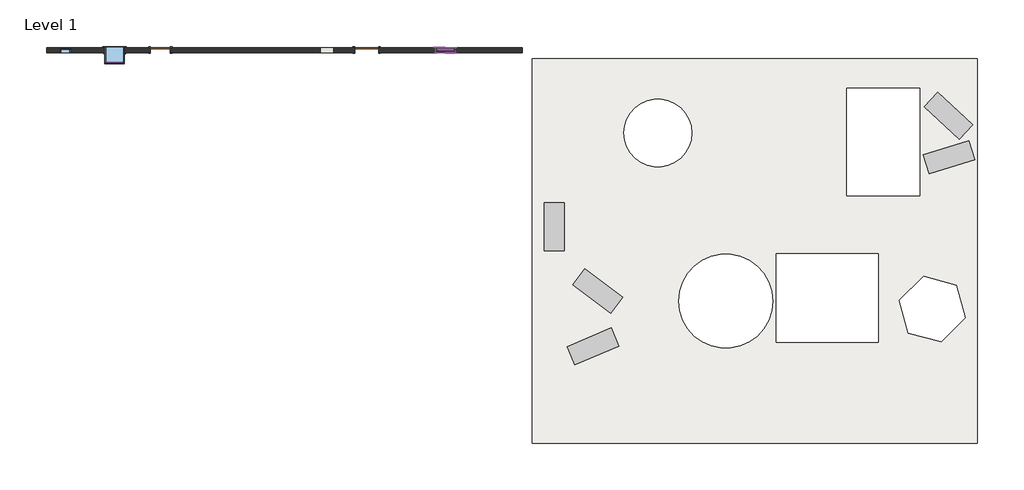
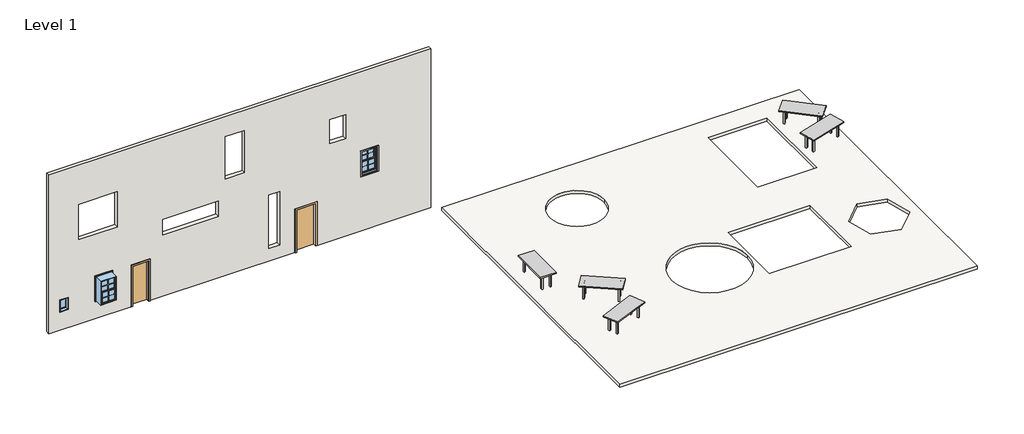
# One storey: 8 furniture elements, 8 proxies, 3 windows, 2 doors, 2 slabs, 1 wall.
"""IFC4 building model written with IfcOpenShell, lengths in millimetres."""

import ifcopenshell
import ifcopenshell.guid

model = None  # the IFC model being written
_history = None  # IfcOwnerHistory: only IFC2X3 demands one
_inside = {}  # id of a spatial element -> (the spatial element, [elements in it])
_under = {}  # id of a project, library or spatial element -> (it, [spatial elements below it])
_declared = {}  # id of a project -> (the project, [libraries it declares])
_typed = {}  # id of a type object -> (the type object, [elements of that type])
_made_of = {}  # id of a material, layer set ... -> (it, [elements and type objects made of it])


def new_model(schema):
    """Start an empty IFC model of exactly this schema.

    Asked for "IFC4X3", IfcOpenShell would pick the latest addendum, in which some entities
    have other attributes; the version numbers below select the first issue.
    IFC2X3 requires an IfcOwnerHistory on every rooted entity: one is made here for all.
    """
    global model, _history
    if schema == "IFC4X3":
        model = ifcopenshell.file(schema_version=(4, 3, 0, 0))
    else:
        model = ifcopenshell.file(schema=schema)
    _inside.clear()
    _under.clear()
    _declared.clear()
    _typed.clear()
    _made_of.clear()
    _history = None
    if model.schema == "IFC2X3":
        org = make("IfcOrganization", Name="unknown")
        user = make(
            "IfcPersonAndOrganization",
            ThePerson=make("IfcPerson", FamilyName="unknown"),
            TheOrganization=org,
        )
        app = make(
            "IfcApplication",
            ApplicationDeveloper=org,
            Version="unknown",
            ApplicationFullName="unknown",
            ApplicationIdentifier="unknown",
        )
        _history = make(
            "IfcOwnerHistory",
            OwningUser=user,
            OwningApplication=app,
            ChangeAction="ADDED",
            CreationDate=0,
        )
    return model


def make(cls, **values):
    """One entity of the class cls with the attributes given. An attribute that is None is left unset."""
    return model.create_entity(
        cls, **{name: value for name, value in values.items() if value is not None}
    )


def rooted(cls, **values):
    """An entity with a GlobalId (a new one), such as an element, a storey or a relation."""
    return make(cls, GlobalId=ifcopenshell.guid.new(), OwnerHistory=_history, **values)


def si_unit(unit_type, name, prefix=None):
    """IfcSIUnit, for example si_unit("LENGTHUNIT", "METRE", prefix="MILLI")."""
    return make("IfcSIUnit", UnitType=unit_type, Prefix=prefix, Name=name)


def assignment(units):
    """IfcUnitAssignment: the units of a project."""
    return None if units is None else make("IfcUnitAssignment", Units=units)


def point(xyz):
    """IfcCartesianPoint."""
    return None if xyz is None else make("IfcCartesianPoint", Coordinates=xyz)


def direction(xyz):
    """IfcDirection."""
    return None if xyz is None else make("IfcDirection", DirectionRatios=xyz)


def frame(location, z_axis=None, x_axis=None):
    """IfcAxis2Placement3D, a coordinate frame: its origin and axes. An axis left out is left unset."""
    return make(
        "IfcAxis2Placement3D",
        Location=point(location),
        Axis=direction(z_axis),
        RefDirection=direction(x_axis),
    )


def frame_2d(location, x_axis=None):
    """IfcAxis2Placement2D, a coordinate frame in the plane: its origin and x axis."""
    return make(
        "IfcAxis2Placement2D", Location=point(location), RefDirection=direction(x_axis)
    )


def origin():
    """The frame at (0, 0, 0) with its axes left unset."""
    return frame((0.0, 0.0, 0.0))


def origin_with_axes():
    """The frame at (0, 0, 0) with the z axis (0, 0, 1) and the x axis (1, 0, 0) written out."""
    return frame((0.0, 0.0, 0.0), z_axis=(0.0, 0.0, 1.0), x_axis=(1.0, 0.0, 0.0))


def place(relative_to, where):
    """IfcLocalPlacement: puts the frame where relative to a parent placement (None: the world)."""
    return make(
        "IfcLocalPlacement", PlacementRelTo=relative_to, RelativePlacement=where
    )


def context(
    kind, dimensions, precision=None, world=None, true_north=None, identifier=None
):
    """IfcGeometricRepresentationContext, for example the 3D "Model" context."""
    return make(
        "IfcGeometricRepresentationContext",
        ContextIdentifier=identifier,
        ContextType=kind,
        CoordinateSpaceDimension=dimensions,
        Precision=precision,
        WorldCoordinateSystem=world,
        TrueNorth=true_north,
    )


def project(units=None, contexts=None):
    """IfcProject with its units and contexts."""
    return rooted(
        "IfcProject",
        Name="project",
        RepresentationContexts=contexts,
        UnitsInContext=assignment(units),
    )


def spatial(cls, under=None, at=None, **own):
    """A site, building, storey or space (cls), placed at a placement, below another one or the project."""
    s = rooted(cls, ObjectPlacement=at, **own)
    if under is not None:
        _under.setdefault(under.id(), (under, []))[1].append(s)
    return s


def polyline(points):
    """IfcPolyline through the points."""
    return make("IfcPolyline", Points=[point(p) for p in points])


def circle_curve(where, radius):
    """IfcCircle in the frame where."""
    return make("IfcCircle", Position=where, Radius=radius)


def trimmed(basis, trim1, trim2, sense, master):
    """IfcTrimmedCurve: the piece of a basis curve between two trims."""
    return make(
        "IfcTrimmedCurve",
        BasisCurve=basis,
        Trim1=trim1,
        Trim2=trim2,
        SenseAgreement=sense,
        MasterRepresentation=master,
    )


def segment(curve, same_sense, transition):
    """IfcCompositeCurveSegment."""
    return make(
        "IfcCompositeCurveSegment",
        Transition=transition,
        SameSense=same_sense,
        ParentCurve=curve,
    )


def composite_curve(segments, self_intersect=None):
    """IfcCompositeCurve: segments joined end to end."""
    return make("IfcCompositeCurve", Segments=segments, SelfIntersect=self_intersect)


def outline(outer, holes=None, kind="AREA"):
    """IfcArbitraryClosedProfileDef: a profile drawn as a closed curve; with holes, ...WithVoids."""
    if holes is None:
        return make("IfcArbitraryClosedProfileDef", ProfileType=kind, OuterCurve=outer)
    return make(
        "IfcArbitraryProfileDefWithVoids",
        ProfileType=kind,
        OuterCurve=outer,
        InnerCurves=holes,
    )


def extrude(swept, where, along, depth):
    """IfcExtrudedAreaSolid: the profile swept, set in the frame where, extruded along a direction by depth."""
    return make(
        "IfcExtrudedAreaSolid",
        SweptArea=swept,
        Position=where,
        ExtrudedDirection=direction(along),
        Depth=depth,
    )


def shape(context_of_items, identifier, shape_type, items):
    """IfcShapeRepresentation: the items that make up one representation, for example the "Body"."""
    return make(
        "IfcShapeRepresentation",
        ContextOfItems=context_of_items,
        RepresentationIdentifier=identifier,
        RepresentationType=shape_type,
        Items=items,
    )


def source(mapping_origin, context_of_items, identifier, shape_type, items):
    """IfcRepresentationMap: a shape defined once, which mapped items show again and again."""
    return make(
        "IfcRepresentationMap",
        MappingOrigin=mapping_origin,
        MappedRepresentation=shape(context_of_items, identifier, shape_type, items),
    )


def transform(
    local_origin,
    x_axis=None,
    y_axis=None,
    z_axis=None,
    scale=None,
    scale2=None,
    scale3=None,
    uniform=True,
):
    """IfcCartesianTransformationOperator3D, or its non-uniform kind. x_axis, y_axis, z_axis: its Axis1, 2, 3."""
    if uniform:
        return make(
            "IfcCartesianTransformationOperator3D",
            Axis1=direction(x_axis),
            Axis2=direction(y_axis),
            LocalOrigin=point(local_origin),
            Scale=scale,
            Axis3=direction(z_axis),
        )
    return make(
        "IfcCartesianTransformationOperator3DnonUniform",
        Axis1=direction(x_axis),
        Axis2=direction(y_axis),
        LocalOrigin=point(local_origin),
        Scale=scale,
        Axis3=direction(z_axis),
        Scale2=scale2,
        Scale3=scale3,
    )


def mapped(mapping_source, mapping_target):
    """IfcMappedItem: shows the shape of a source again, moved by a transform."""
    return make(
        "IfcMappedItem", MappingSource=mapping_source, MappingTarget=mapping_target
    )


def made_of(thing, what):
    """Note that an element or type object is made of a material, layer set ...; save() writes the relation."""
    if what is not None:
        _made_of.setdefault(what.id(), (what, []))[1].append(thing)
    return thing


def element(
    cls,
    number,
    at=None,
    inside=None,
    cuts=None,
    type_object=None,
    material=None,
    context=None,
    identifier="Body",
    shape_type=None,
    held_by="IfcProductDefinitionShape",
    body=None,
    shapes=None,
    **own,
):
    """One element of the class cls, such as IfcWall. Its Tag is "e" and its number.

    at: its placement. inside: the storey or other place that contains it. cuts: it is an
    opening in that element (IfcRelVoidsElement). A single representation is given by context,
    identifier, shape_type and body (its items); several are given by shapes. held_by: the class
    of the entity that holds the representations. save() writes the other relations.
    """
    e = rooted(cls, Tag="e%d" % number, ObjectPlacement=at, **own)
    if body is not None:
        shapes = [shape(context, identifier, shape_type, body)]
    if shapes is not None:
        e.Representation = make(held_by, Representations=shapes)
    if inside is not None:
        _inside.setdefault(inside.id(), (inside, []))[1].append(e)
    if cuts is not None:
        rooted(
            "IfcRelVoidsElement", RelatingBuildingElement=cuts, RelatedOpeningElement=e
        )
    if type_object is not None:
        _typed.setdefault(type_object.id(), (type_object, []))[1].append(e)
    return made_of(e, material)


def aggregate(whole, parts):
    """IfcRelAggregates: a whole, such as a stair, and the parts it consists of."""
    return rooted("IfcRelAggregates", RelatingObject=whole, RelatedObjects=parts)


def save(model, path):
    """Write the relations noted so far, then the file.

    IfcRelAggregates (storeys below a building ...), IfcRelContainedInSpatialStructure (elements
    in a storey), IfcRelDefinesByType, IfcRelAssociatesMaterial and IfcRelDeclares: one each for
    every whole, place, type object, material and project.
    """
    for whole, parts in _under.values():
        aggregate(whole, parts)
    for where, things in _inside.values():
        rooted(
            "IfcRelContainedInSpatialStructure",
            RelatedElements=things,
            RelatingStructure=where,
        )
    for kind, things in _typed.values():
        rooted("IfcRelDefinesByType", RelatedObjects=things, RelatingType=kind)
    for what, things in _made_of.values():
        rooted("IfcRelAssociatesMaterial", RelatedObjects=things, RelatingMaterial=what)
    for by, libraries in _declared.values():
        rooted("IfcRelDeclares", RelatingContext=by, RelatedDefinitions=libraries)
    model.write(path)


def m_muntin_pattern_2x2_m_muntin_pattern_2x2_aaec3afb(model_context):
    return source(origin(), model_context, "Body", "SweptSolid", [
        extrude(outline(polyline([(257.1375, -6.35), (257.1375, -298.8), (244.4375, -298.8), (244.4375, -6.35), (0.0, -6.35), (0.0, 6.35), (244.4375, 6.35), (244.4375, 298.8), (257.1375, 298.8), (257.1375, 6.35), (501.575, 6.35), (501.575, -6.35), (257.1375, -6.35)])), frame((0.0, 9.525, 0.0), z_axis=(0.0, 1.0, 0.0), x_axis=(0.0, 0.0, 1.0)), (0.0, 0.0, 1.0), 12.7),
        extrude(outline(polyline([(257.1375, -6.35), (257.1375, -298.8), (244.4375, -298.8), (244.4375, -6.35), (0.0, -6.35), (0.0, 6.35), (244.4375, 6.35), (244.4375, 298.8), (257.1375, 298.8), (257.1375, 6.35), (501.575, 6.35), (501.575, -6.35), (257.1375, -6.35)])), frame((0.0, -22.225, 0.0), z_axis=(0.0, 1.0, 0.0), x_axis=(0.0, 0.0, 1.0)), (0.0, 0.0, 1.0), 12.7),
    ])


def m_trim_window_exterior_flat_with_sill_e7ff6350(model_context):
    return source(origin(), model_context, "Body", "SweptSolid", [
        extrude(outline(polyline([(435.0, -1220.4323709), (435.0, -1280.4323709), (-435.0, -1280.4323709), (-435.0, -1220.4323709), (435.0, -1220.4323709)])), origin_with_axes(), (0.0, 0.0, 1.0), 19.05),
        extrude(outline(polyline([(-1230.0, 38.1), (-1202.4580645, 38.1), (-1200.0, 19.05), (-1200.0, 0.0), (-1220.4323709, 0.0), (-1220.4323709, 19.05), (-1230.0, 19.05), (-1230.0, 38.1)])), frame((-447.7, 0.0, 0.0), z_axis=(1.0, 0.0, 0.0), x_axis=(0.0, 1.0, 0.0)), (0.0, 0.0, 1.0), 895.4),
        extrude(outline(polyline([(-435.0, 60.0), (435.0, 60.0), (435.0, -1200.0), (375.0, -1200.0), (375.0, 0.0), (-375.0, 0.0), (-375.0, -1200.0), (-435.0, -1200.0), (-435.0, 60.0)])), origin_with_axes(), (0.0, 0.0, 1.0), 19.05),
    ])


def m_trim_window_interior_flat_picture_frame_31bd2320(model_context):
    return source(origin(), model_context, "Body", "SweptSolid", [
        extrude(outline(polyline([(422.3, 47.3), (422.3, -1247.3), (-422.3, -1247.3), (-422.3, 47.3), (422.3, 47.3)]), holes=[polyline([(362.3, -12.7), (-362.3, -12.7), (-362.3, -1187.3), (362.3, -1187.3), (362.3, -12.7)])]), origin_with_axes(), (0.0, 0.0, 1.0), 30.0),
    ])


def m_single_flush_0762_x_2032mm_0c256fab(model_context):
    return source(origin(), model_context, "Body", "SweptSolid", [
        extrude(outline(polyline([(2108.0, -457.0), (0.0, -457.0), (0.0, -381.0), (2032.0, -381.0), (2032.0, 381.0), (0.0, 381.0), (0.0, 457.0), (2108.0, 457.0), (2108.0, -457.0)])), frame((0.0, 100.0, 0.0), z_axis=(0.0, 1.0, 0.0), x_axis=(0.0, 0.0, 1.0)), (0.0, 0.0, 1.0), 25.0),
        extrude(outline(polyline([(2108.0, 457.0), (2108.0, -457.0), (0.0, -457.0), (0.0, -381.0), (2032.0, -381.0), (2032.0, 381.0), (0.0, 381.0), (0.0, 457.0), (2108.0, 457.0)])), frame((0.0, -125.0, 0.0), z_axis=(0.0, 1.0, 0.0), x_axis=(0.0, 0.0, 1.0)), (0.0, 0.0, 1.0), 25.0),
        extrude(outline(polyline([(381.0, 49.0), (-381.0, 49.0), (-381.0, 100.0), (381.0, 100.0), (381.0, 49.0)])), origin_with_axes(), (0.0, 0.0, 1.0), 2032.0),
    ])


def m_single_flush_0915_x_2134mm_727434cd(model_context):
    return source(origin(), model_context, "Body", "SweptSolid", [
        extrude(outline(polyline([(2210.0, -533.5), (0.0, -533.5), (0.0, -457.5), (2134.0, -457.5), (2134.0, 457.5), (0.0, 457.5), (0.0, 533.5), (2210.0, 533.5), (2210.0, -533.5)])), frame((0.0, -125.0, 0.0), z_axis=(0.0, 1.0, 0.0), x_axis=(0.0, 0.0, 1.0)), (0.0, 0.0, 1.0), 25.0),
        extrude(outline(polyline([(2210.0, 533.5), (2210.0, -533.5), (0.0, -533.5), (0.0, -457.5), (2134.0, -457.5), (2134.0, 457.5), (0.0, 457.5), (0.0, 533.5), (2210.0, 533.5)])), frame((0.0, 100.0, 0.0), z_axis=(0.0, 1.0, 0.0), x_axis=(0.0, 0.0, 1.0)), (0.0, 0.0, 1.0), 25.0),
        extrude(outline(polyline([(457.5, -49.0), (457.5, -100.0), (-457.5, -100.0), (-457.5, -49.0), (457.5, -49.0)])), origin_with_axes(), (0.0, 0.0, 1.0), 2134.0),
    ])


def m_table_rectangular_1830_x_0762mm_a0b3b7a0(model_context):
    return source(origin(), model_context, "Body", "SweptSolid", [
        extrude(outline(polyline([(699.1, 190.5), (699.1, 165.1), (-699.1, 165.1), (-699.1, 190.5), (699.1, 190.5)])), frame((0.0, 0.0, 609.6), z_axis=(0.0, 0.0, 1.0), x_axis=(1.0, 0.0, 0.0)), (0.0, 0.0, 1.0), 101.6),
        extrude(outline(polyline([(699.1, -190.5), (-699.1, -190.5), (-699.1, -165.1), (699.1, -165.1), (699.1, -190.5)])), frame((0.0, 0.0, 609.6), z_axis=(0.0, 0.0, 1.0), x_axis=(1.0, 0.0, 0.0)), (0.0, 0.0, 1.0), 101.6),
        extrude(outline(polyline([(-711.8, -165.1), (-737.2, -165.1), (-737.2, 165.1), (-711.8, 165.1), (-711.8, -165.1)])), frame((0.0, 0.0, 609.6), z_axis=(0.0, 0.0, 1.0), x_axis=(1.0, 0.0, 0.0)), (0.0, 0.0, 1.0), 101.6),
        extrude(outline(polyline([(711.8, -165.1), (711.8, 165.1), (737.2, 165.1), (737.2, -165.1), (711.8, -165.1)])), frame((0.0, 0.0, 609.6), z_axis=(0.0, 0.0, 1.0), x_axis=(1.0, 0.0, 0.0)), (0.0, 0.0, 1.0), 101.6),
        extrude(outline(polyline([(915.0, 381.0), (915.0, -381.0), (-915.0, -381.0), (-915.0, 381.0), (915.0, 381.0)])), frame((0.0, 0.0, 711.2), z_axis=(0.0, 0.0, 1.0), x_axis=(1.0, 0.0, 0.0)), (0.0, 0.0, 1.0), 50.8),
        extrude(outline(polyline([(-699.1, 228.6), (-699.1, 165.1), (-762.6, 165.1), (-762.6, 228.6), (-699.1, 228.6)])), origin_with_axes(), (0.0, 0.0, 1.0), 711.2),
        extrude(outline(polyline([(699.1, 228.6), (762.6, 228.6), (762.6, 165.1), (699.1, 165.1), (699.1, 228.6)])), origin_with_axes(), (0.0, 0.0, 1.0), 711.2),
        extrude(outline(polyline([(-699.1, -228.6), (-762.6, -228.6), (-762.6, -165.1), (-699.1, -165.1), (-699.1, -228.6)])), origin_with_axes(), (0.0, 0.0, 1.0), 711.2),
        extrude(outline(polyline([(699.1, -228.6), (699.1, -165.1), (762.6, -165.1), (762.6, -228.6), (699.1, -228.6)])), origin_with_axes(), (0.0, 0.0, 1.0), 711.2),
    ])


def m_table_rectangular_1830_x_0762mm_ec068ed4(model_context):
    return source(origin(), model_context, "Body", "SweptSolid", [
        extrude(outline(polyline([(699.1, -190.5), (-699.1, -190.5), (-699.1, -165.1), (699.1, -165.1), (699.1, -190.5)])), frame((0.0, 0.0, 609.6), z_axis=(0.0, 0.0, 1.0), x_axis=(1.0, 0.0, 0.0)), (0.0, 0.0, 1.0), 101.6),
        extrude(outline(polyline([(699.1, 190.5), (699.1, 165.1), (-699.1, 165.1), (-699.1, 190.5), (699.1, 190.5)])), frame((0.0, 0.0, 609.6), z_axis=(0.0, 0.0, 1.0), x_axis=(1.0, 0.0, 0.0)), (0.0, 0.0, 1.0), 101.6),
        extrude(outline(polyline([(-711.8, 165.1), (-711.8, -165.1), (-737.2, -165.1), (-737.2, 165.1), (-711.8, 165.1)])), frame((0.0, 0.0, 609.6), z_axis=(0.0, 0.0, 1.0), x_axis=(1.0, 0.0, 0.0)), (0.0, 0.0, 1.0), 101.6),
        extrude(outline(polyline([(711.8, 165.1), (737.2, 165.1), (737.2, -165.1), (711.8, -165.1), (711.8, 165.1)])), frame((0.0, 0.0, 609.6), z_axis=(0.0, 0.0, 1.0), x_axis=(1.0, 0.0, 0.0)), (0.0, 0.0, 1.0), 101.6),
        extrude(outline(polyline([(915.0, -381.0), (-915.0, -381.0), (-915.0, 381.0), (915.0, 381.0), (915.0, -381.0)])), frame((0.0, 0.0, 711.2), z_axis=(0.0, 0.0, 1.0), x_axis=(1.0, 0.0, 0.0)), (0.0, 0.0, 1.0), 50.8),
        extrude(outline(polyline([(-699.1, -228.6), (-762.6, -228.6), (-762.6, -165.1), (-699.1, -165.1), (-699.1, -228.6)])), origin_with_axes(), (0.0, 0.0, 1.0), 711.2),
        extrude(outline(polyline([(699.1, -228.6), (699.1, -165.1), (762.6, -165.1), (762.6, -228.6), (699.1, -228.6)])), origin_with_axes(), (0.0, 0.0, 1.0), 711.2),
        extrude(outline(polyline([(-699.1, 228.6), (-699.1, 165.1), (-762.6, 165.1), (-762.6, 228.6), (-699.1, 228.6)])), origin_with_axes(), (0.0, 0.0, 1.0), 711.2),
        extrude(outline(polyline([(699.1, 228.6), (762.6, 228.6), (762.6, 165.1), (699.1, 165.1), (699.1, 228.6)])), origin_with_axes(), (0.0, 0.0, 1.0), 711.2),
    ])


def m_fixed_0406_x_0610mm_8205b201(model_context):
    return source(origin(), model_context, "Body", "SweptSolid", [
        extrude(outline(polyline([(-140.0, 78.0), (140.0, 78.0), (140.0, 66.0), (-140.0, 66.0), (-140.0, 78.0)])), frame((0.0, 0.0, 978.0), z_axis=(0.0, 0.0, 1.0), x_axis=(1.0, 0.0, 0.0)), (0.0, 0.0, 1.0), 484.0),
        extrude(outline(polyline([(1506.0, -184.0), (934.0, -184.0), (934.0, 184.0), (1506.0, 184.0), (1506.0, -184.0)]), holes=[polyline([(1462.0, -140.0), (1462.0, 140.0), (978.0, 140.0), (978.0, -140.0), (1462.0, -140.0)])]), frame((0.0, 50.0, 0.0), z_axis=(0.0, 1.0, 0.0), x_axis=(0.0, 0.0, 1.0)), (0.0, 0.0, 1.0), 44.0),
        extrude(outline(polyline([(1525.0, -203.0), (915.0, -203.0), (915.0, 203.0), (1525.0, 203.0), (1525.0, -203.0)]), holes=[polyline([(1506.0, -184.0), (1506.0, 184.0), (934.0, 184.0), (934.0, -184.0), (1506.0, -184.0)])]), frame((0.0, 50.0, 0.0), z_axis=(0.0, 1.0, 0.0), x_axis=(0.0, 0.0, 1.0)), (0.0, 0.0, 1.0), 63.0),
        extrude(outline(polyline([(1525.0, -203.0), (915.0, -203.0), (915.0, 203.0), (1525.0, 203.0), (1525.0, -203.0)]), holes=[polyline([(1493.0, -171.0), (1493.0, 171.0), (947.0, 171.0), (947.0, -171.0), (1493.0, -171.0)])]), frame((0.0, -87.0, 0.0), z_axis=(0.0, 1.0, 0.0), x_axis=(0.0, 0.0, 1.0)), (0.0, 0.0, 1.0), 137.0),
    ])


def m_window_double_hung_750_x_1200mm_e21ea802(model_context):
    return source(origin(), model_context, "Body", "SweptSolid", [
        extrude(outline(polyline([(298.8, -469.85), (298.8, -476.2), (-298.8, -476.2), (-298.8, -469.85), (298.8, -469.85)])), frame((0.0, 0.0, 990.6), z_axis=(0.0, 0.0, 1.0), x_axis=(1.0, 0.0, 0.0)), (0.0, 0.0, 1.0), 501.575),
        extrude(outline(polyline([(-298.8, -482.55), (298.8, -482.55), (298.8, -488.9), (-298.8, -488.9), (-298.8, -482.55)])), frame((0.0, 0.0, 990.6), z_axis=(0.0, 0.0, 1.0), x_axis=(1.0, 0.0, 0.0)), (0.0, 0.0, 1.0), 501.575),
        extrude(outline(polyline([(298.8, -425.4), (298.8, -431.75), (-298.8, -431.75), (-298.8, -425.4), (298.8, -425.4)])), frame((0.0, 0.0, 1536.625), z_axis=(0.0, 0.0, 1.0), x_axis=(1.0, 0.0, 0.0)), (0.0, 0.0, 1.0), 501.575),
        extrude(outline(polyline([(-298.8, -438.1), (298.8, -438.1), (298.8, -444.45), (-298.8, -444.45), (-298.8, -438.1)])), frame((0.0, 0.0, 1536.625), z_axis=(0.0, 0.0, 1.0), x_axis=(1.0, 0.0, 0.0)), (0.0, 0.0, 1.0), 501.575),
        extrude(outline(polyline([(1536.625, -343.25), (946.15, -343.25), (946.15, 343.25), (1536.625, 343.25), (1536.625, -343.25)]), holes=[polyline([(1492.175, 298.8), (990.6, 298.8), (990.6, -298.8), (1492.175, -298.8), (1492.175, 298.8)])]), frame((0.0, -501.6, 0.0), z_axis=(0.0, 1.0, 0.0), x_axis=(0.0, 0.0, 1.0)), (0.0, 0.0, 1.0), 44.45),
        extrude(outline(polyline([(2082.65, -343.25), (1492.175, -343.25), (1492.175, 343.25), (2082.65, 343.25), (2082.65, -343.25)]), holes=[polyline([(2038.2, 298.8), (1536.625, 298.8), (1536.625, -298.8), (2038.2, -298.8), (2038.2, 298.8)])]), frame((0.0, -457.15, 0.0), z_axis=(0.0, 1.0, 0.0), x_axis=(0.0, 0.0, 1.0)), (0.0, 0.0, 1.0), 44.45),
        extrude(outline(polyline([(2114.4, -375.0), (914.4, -375.0), (914.4, 375.0), (2114.4, 375.0), (2114.4, -375.0)]), holes=[polyline([(2082.65, 343.25), (946.15, 343.25), (946.15, -343.25), (2082.65, -343.25), (2082.65, 343.25)])]), frame((0.0, -514.3, 0.0), z_axis=(0.0, 1.0, 0.0), x_axis=(0.0, 0.0, 1.0)), (0.0, 0.0, 1.0), 633.35),
    ])


def m_window_double_hung_750_x_1200mm_41070976(model_context):
    return source(origin(), model_context, "Body", "SweptSolid", [
        extrude(outline(polyline([(298.8, 30.15), (298.8, 23.8), (-298.8, 23.8), (-298.8, 30.15), (298.8, 30.15)])), frame((0.0, 0.0, 990.6), z_axis=(0.0, 0.0, 1.0), x_axis=(1.0, 0.0, 0.0)), (0.0, 0.0, 1.0), 501.575),
        extrude(outline(polyline([(-298.8, 17.45), (298.8, 17.45), (298.8, 11.1), (-298.8, 11.1), (-298.8, 17.45)])), frame((0.0, 0.0, 990.6), z_axis=(0.0, 0.0, 1.0), x_axis=(1.0, 0.0, 0.0)), (0.0, 0.0, 1.0), 501.575),
        extrude(outline(polyline([(298.8, 74.6), (298.8, 68.25), (-298.8, 68.25), (-298.8, 74.6), (298.8, 74.6)])), frame((0.0, 0.0, 1536.625), z_axis=(0.0, 0.0, 1.0), x_axis=(1.0, 0.0, 0.0)), (0.0, 0.0, 1.0), 501.575),
        extrude(outline(polyline([(-298.8, 61.9), (298.8, 61.9), (298.8, 55.55), (-298.8, 55.55), (-298.8, 61.9)])), frame((0.0, 0.0, 1536.625), z_axis=(0.0, 0.0, 1.0), x_axis=(1.0, 0.0, 0.0)), (0.0, 0.0, 1.0), 501.575),
        extrude(outline(polyline([(1536.625, -343.25), (946.15, -343.25), (946.15, 343.25), (1536.625, 343.25), (1536.625, -343.25)]), holes=[polyline([(1492.175, 298.8), (990.6, 298.8), (990.6, -298.8), (1492.175, -298.8), (1492.175, 298.8)])]), frame((0.0, -1.6, 0.0), z_axis=(0.0, 1.0, 0.0), x_axis=(0.0, 0.0, 1.0)), (0.0, 0.0, 1.0), 44.45),
        extrude(outline(polyline([(2082.65, -343.25), (1492.175, -343.25), (1492.175, 343.25), (2082.65, 343.25), (2082.65, -343.25)]), holes=[polyline([(2038.2, 298.8), (1536.625, 298.8), (1536.625, -298.8), (2038.2, -298.8), (2038.2, 298.8)])]), frame((0.0, 42.85, 0.0), z_axis=(0.0, 1.0, 0.0), x_axis=(0.0, 0.0, 1.0)), (0.0, 0.0, 1.0), 44.45),
        extrude(outline(polyline([(2114.4, -375.0), (914.4, -375.0), (914.4, 375.0), (2114.4, 375.0), (2114.4, -375.0)]), holes=[polyline([(2082.65, 343.25), (946.15, 343.25), (946.15, -343.25), (2082.65, -343.25), (2082.65, 343.25)])]), frame((0.0, -14.3, 0.0), z_axis=(0.0, 1.0, 0.0), x_axis=(0.0, 0.0, 1.0)), (0.0, 0.0, 1.0), 133.35),
        extrude(outline(polyline([(2114.4, 375.0), (2114.4, -375.0), (914.4, -375.0), (914.4, 375.0), (2114.4, 375.0)]), holes=[polyline([(2095.35, 355.95), (933.45, 355.95), (933.45, -355.95), (2095.35, -355.95), (2095.35, 355.95)])]), frame((0.0, -100.0, 0.0), z_axis=(0.0, 1.0, 0.0), x_axis=(0.0, 0.0, 1.0)), (0.0, 0.0, 1.0), 85.7),
    ])


model = new_model("IFC4")

# Units and contexts
model_context = context("Model", 3, world=origin())
ifc_project = project(units=[si_unit("LENGTHUNIT", "METRE", prefix="MILLI")], contexts=[model_context])

# Site, building, storey
site = spatial("IfcSite", under=ifc_project)
building = spatial("IfcBuilding", under=site)
storey = spatial("IfcBuildingStorey", under=building, Name="Level 1", Elevation=0.0)

# Proxies
placement = place(None, origin())
m_muntin_pattern_2x2_m_muntin_pattern_2x2_shape = m_muntin_pattern_2x2_m_muntin_pattern_2x2_aaec3afb(model_context)
element("IfcBuildingElementProxy", 1, Name="M_Muntin Pattern_2x2 : M_Muntin Pattern_2x2", ObjectType="M_Muntin Pattern_2x2 : M_Muntin Pattern_2x2", at=placement, inside=storey, context=model_context, shape_type="MappedRepresentation", body=[
    mapped(m_muntin_pattern_2x2_m_muntin_pattern_2x2_shape, transform((-13755.2543844, 2099.5505832, 3404.9440493), x_axis=(1.0, 0.0, 0.0), y_axis=(0.0, 1.0, 0.0), z_axis=(0.0, 0.0, 1.0))),
])
element("IfcBuildingElementProxy", 2, Name="M_Muntin Pattern_2x2 : M_Muntin Pattern_2x2", ObjectType="M_Muntin Pattern_2x2 : M_Muntin Pattern_2x2", at=placement, inside=storey, context=model_context, shape_type="MappedRepresentation", body=[
    mapped(m_muntin_pattern_2x2_m_muntin_pattern_2x2_shape, transform((-13755.2543844, 2055.1005832, 2858.9190493), x_axis=(1.0, 0.0, 0.0), y_axis=(0.0, 1.0, 0.0), z_axis=(0.0, 0.0, 1.0))),
])
element("IfcBuildingElementProxy", 3, Name="M_Muntin Pattern_2x2 : M_Muntin Pattern_2x2", ObjectType="M_Muntin Pattern_2x2 : M_Muntin Pattern_2x2", at=placement, inside=storey, context=model_context, shape_type="MappedRepresentation", body=[
    mapped(m_muntin_pattern_2x2_m_muntin_pattern_2x2_shape, transform((-26415.5284847, 1599.5505832, 1536.625), x_axis=(1.0, 0.0, 0.0), y_axis=(0.0, 1.0, 0.0), z_axis=(0.0, 0.0, 1.0))),
])
element("IfcBuildingElementProxy", 4, Name="M_Muntin Pattern_2x2 : M_Muntin Pattern_2x2", ObjectType="M_Muntin Pattern_2x2 : M_Muntin Pattern_2x2", at=placement, inside=storey, context=model_context, shape_type="MappedRepresentation", body=[
    mapped(m_muntin_pattern_2x2_m_muntin_pattern_2x2_shape, transform((-26415.5284847, 1555.1005832, 990.6), x_axis=(1.0, 0.0, 0.0), y_axis=(0.0, 1.0, 0.0), z_axis=(0.0, 0.0, 1.0))),
])
m_trim_window_exterior_flat_with_sill_shape = m_trim_window_exterior_flat_with_sill_e7ff6350(model_context)
element("IfcBuildingElementProxy", 5, Name="M_Trim-Window-Exterior-Flat : with Sill", ObjectType="M_Trim-Window-Exterior-Flat : with Sill", at=placement, inside=storey, context=model_context, shape_type="MappedRepresentation", body=[
    mapped(m_trim_window_exterior_flat_with_sill_shape, transform((-13755.2543844, 2134.4755832, 3982.7190493), x_axis=(-1.0, 0.0, 0.0), y_axis=(0.0, 0.0, 1.0), z_axis=(0.0, 1.0, 0.0))),
])
element("IfcBuildingElementProxy", 6, Name="M_Trim-Window-Exterior-Flat : with Sill", ObjectType="M_Trim-Window-Exterior-Flat : with Sill", at=placement, inside=storey, context=model_context, shape_type="MappedRepresentation", body=[
    mapped(m_trim_window_exterior_flat_with_sill_shape, transform((-26415.5284847, 2134.4755832, 2114.4), x_axis=(-1.0, 0.0, 0.0), y_axis=(0.0, 0.0, 1.0), z_axis=(0.0, 1.0, 0.0))),
])
m_trim_window_interior_flat_picture_frame_shape = m_trim_window_interior_flat_picture_frame_31bd2320(model_context)
element("IfcBuildingElementProxy", 7, Name="M_Trim-Window-Interior-Flat : Picture Frame", ObjectType="M_Trim-Window-Interior-Flat : Picture Frame", at=placement, inside=storey, context=model_context, shape_type="MappedRepresentation", body=[
    mapped(m_trim_window_interior_flat_picture_frame_shape, transform((-13755.2543844, 1934.4755832, 3982.7190493), x_axis=(1.0, 0.0, 0.0), y_axis=(0.0, 0.0, 1.0), z_axis=(0.0, -1.0, 0.0))),
])
element("IfcBuildingElementProxy", 8, Name="M_Trim-Window-Interior-Flat : Picture Frame", ObjectType="M_Trim-Window-Interior-Flat : Picture Frame", at=placement, inside=storey, context=model_context, shape_type="MappedRepresentation", body=[
    mapped(m_trim_window_interior_flat_picture_frame_shape, transform((-26415.5284847, 1934.4755832, 2114.4), x_axis=(1.0, 0.0, 0.0), y_axis=(0.0, 0.0, 1.0), z_axis=(0.0, -1.0, 0.0))),
])

# Doors
m_single_flush_0762_x_2032mm_shape = m_single_flush_0762_x_2032mm_0c256fab(model_context)
element("IfcDoor", 9, ObjectType="M_Single-Flush : 0762 x 2032mm", at=placement, inside=storey, context=model_context, shape_type="MappedRepresentation", body=[
    mapped(m_single_flush_0762_x_2032mm_shape, transform((-24659.5284847, 2034.4755832, 0.0), x_axis=(1.0, 0.0, 0.0), y_axis=(0.0, 1.0, 0.0), z_axis=(0.0, 0.0, 1.0))),
])
m_single_flush_0915_x_2134mm_shape = m_single_flush_0915_x_2134mm_727434cd(model_context)
element("IfcDoor", 10, ObjectType="M_Single-Flush : 0915 x 2134mm", at=placement, inside=storey, context=model_context, shape_type="MappedRepresentation", body=[
    mapped(m_single_flush_0915_x_2134mm_shape, transform((-16774.8897659, 2034.4755832, 0.0), x_axis=(-1.0, 0.0, 0.0), y_axis=(0.0, -1.0, 0.0), z_axis=(0.0, 0.0, 1.0))),
])

# Furniture
m_table_rectangular_1830_x_0762mm_shape = m_table_rectangular_1830_x_0762mm_a0b3b7a0(model_context)
element("IfcFurniture", 11, ObjectType="M_Table-Rectangular : 1830 x 0762mm", at=placement, inside=storey, context=model_context, shape_type="MappedRepresentation", body=[
    mapped(m_table_rectangular_1830_x_0762mm_shape, transform((-7934.3891602, -7176.9575195, 0.0), x_axis=(0.7986354897314345, -0.6018150501121021, 0.0), y_axis=(0.6018150501121021, 0.7986354897314345, 0.0), z_axis=(0.0, 0.0, 1.0))),
])
element("IfcFurniture", 12, ObjectType="M_Table-Rectangular : 1830 x 0762mm", at=placement, inside=storey, context=model_context, shape_type="MappedRepresentation", body=[
    mapped(m_table_rectangular_1830_x_0762mm_shape, transform((-9596.1972656, -4723.9775391, 0.0), x_axis=(0.0, 1.0, 0.0), y_axis=(-1.0, 0.0, 0.0), z_axis=(0.0, 0.0, 1.0))),
])
element("IfcFurniture", 13, ObjectType="M_Table-Rectangular : 1830 x 0762mm", at=placement, inside=storey, context=model_context, shape_type="MappedRepresentation", body=[
    mapped(m_table_rectangular_1830_x_0762mm_shape, transform((-8112.0141602, -9301.6689453, 0.0), x_axis=(0.9205048565482237, 0.3907311211960652, 0.0), y_axis=(-0.3907311211960652, 0.9205048565482237, 0.0), z_axis=(0.0, 0.0, 1.0))),
])
element("IfcFurniture", 14, ObjectType="M_Table-Rectangular : 1830 x 0762mm", at=placement, inside=storey, context=model_context, shape_type="MappedRepresentation", body=[
    mapped(m_table_rectangular_1830_x_0762mm_shape, transform((-7934.3891602, -7176.9575195, 0.0), x_axis=(0.7986354897314345, -0.6018150501121021, 0.0), y_axis=(0.6018150501121021, 0.7986354897314345, 0.0), z_axis=(0.0, 0.0, 1.0))),
])
element("IfcFurniture", 15, ObjectType="M_Table-Rectangular : 1830 x 0762mm", at=placement, inside=storey, context=model_context, shape_type="MappedRepresentation", body=[
    mapped(m_table_rectangular_1830_x_0762mm_shape, transform((-9596.1972656, -4723.9775391, 0.0), x_axis=(0.0, 1.0, 0.0), y_axis=(-1.0, 0.0, 0.0), z_axis=(0.0, 0.0, 1.0))),
])
element("IfcFurniture", 16, ObjectType="M_Table-Rectangular : 1830 x 0762mm", at=placement, inside=storey, context=model_context, shape_type="MappedRepresentation", body=[
    mapped(m_table_rectangular_1830_x_0762mm_shape, transform((-8112.0141602, -9301.6689453, 0.0), x_axis=(0.9205048565482237, 0.3907311211960652, 0.0), y_axis=(-0.3907311211960652, 0.9205048565482237, 0.0), z_axis=(0.0, 0.0, 1.0))),
])
m_table_rectangular_1830_x_0762mm_2_shape = m_table_rectangular_1830_x_0762mm_ec068ed4(model_context)
element("IfcFurniture", 17, ObjectType="M_Table-Rectangular : 1830 x 0762mm", at=placement, inside=storey, context=model_context, shape_type="MappedRepresentation", body=[
    mapped(m_table_rectangular_1830_x_0762mm_2_shape, transform((5509.5541992, -2054.6921387, 0.0), x_axis=(-0.9563047576969215, -0.29237169905145133, 0.0), y_axis=(0.29237169905145133, -0.9563047576969215, 0.0), z_axis=(0.0, 0.0, 1.0))),
])
element("IfcFurniture", 18, ObjectType="M_Table-Rectangular : 1830 x 0762mm", at=placement, inside=storey, context=model_context, shape_type="MappedRepresentation", body=[
    mapped(m_table_rectangular_1830_x_0762mm_2_shape, transform((5492.8203125, -469.7512207, 0.0), x_axis=(-0.7313536949478474, 0.6819983672166166, 0.0), y_axis=(-0.6819983672166166, -0.7313536949478474, 0.0), z_axis=(0.0, 0.0, 1.0))),
])

# Slabs
element("IfcSlab", 19, ObjectType="Generic 150mm", at=placement, inside=storey, context=model_context, shape_type="SweptSolid", body=[
    extrude(outline(polyline([(-10438.0920872, 1704.9536342), (6597.1361468, 1704.9536342), (6597.1361468, -12995.0463658), (-10438.0920872, -12995.0463658), (-10438.0920872, 1704.9536342)]), holes=[polyline([(-1096.2822975, -5745.5612839), (-1096.2822975, -9145.5612839), (2803.7177025, -9145.5612839), (2803.7177025, -5745.5612839), (-1096.2822975, -5745.5612839)]), composite_curve([segment(trimmed(circle_curve(frame_2d((-3026.5132944, -7566.8871411)), 1800.0), [point((-1226.5132944, -7566.8871411))], [point((-4826.5132944, -7566.8871411))], True, "CARTESIAN"), True, "CONTINUOUS"), segment(trimmed(circle_curve(frame_2d((-3026.5132944, -7566.8871411)), 1800.0), [point((-4826.5132944, -7566.8871411))], [point((-1226.5132944, -7566.8871411))], True, "CARTESIAN"), True, "CONTINUOUS")], self_intersect=False), polyline([(3950.2905395, -8793.2666419), (5205.9941136, -9129.7314005), (6125.2329292, -8210.492585), (5788.7681706, -6954.7890108), (4533.0645964, -6618.3242522), (3613.8257808, -7537.5630677), (3950.2905395, -8793.2666419)]), polyline([(4397.1361468, 574.3329665), (1597.1361468, 574.3329665), (1597.1361468, -3525.6670335), (4397.1361468, -3525.6670335), (4397.1361468, 574.3329665)]), composite_curve([segment(trimmed(circle_curve(frame_2d((-5632.920233, -1133.8213408)), 1300.0), [point((-4332.920233, -1133.8213408))], [point((-6932.920233, -1133.8213408))], True, "CARTESIAN"), True, "CONTINUOUS"), segment(trimmed(circle_curve(frame_2d((-5632.920233, -1133.8213408)), 1300.0), [point((-6932.920233, -1133.8213408))], [point((-4332.920233, -1133.8213408))], True, "CARTESIAN"), True, "CONTINUOUS")], self_intersect=False)]), frame((0.0, 0.0, -150.0), z_axis=(0.0, 0.0, 1.0), x_axis=(1.0, 0.0, 0.0)), (0.0, 0.0, 1.0), 150.0),
])
element("IfcSlab", 20, ObjectType="Generic 150mm", at=placement, inside=storey, context=model_context, shape_type="SweptSolid", body=[
    extrude(outline(polyline([(-10438.0920872, 1704.9536342), (6597.1361468, 1704.9536342), (6597.1361468, -12995.0463658), (-10438.0920872, -12995.0463658), (-10438.0920872, 1704.9536342)]), holes=[polyline([(-1096.2822975, -5745.5612839), (-1096.2822975, -9145.5612839), (2803.7177025, -9145.5612839), (2803.7177025, -5745.5612839), (-1096.2822975, -5745.5612839)]), composite_curve([segment(trimmed(circle_curve(frame_2d((-3026.5132944, -7566.8871411)), 1800.0), [point((-1226.5132944, -7566.8871411))], [point((-4826.5132944, -7566.8871411))], True, "CARTESIAN"), True, "CONTINUOUS"), segment(trimmed(circle_curve(frame_2d((-3026.5132944, -7566.8871411)), 1800.0), [point((-4826.5132944, -7566.8871411))], [point((-1226.5132944, -7566.8871411))], True, "CARTESIAN"), True, "CONTINUOUS")], self_intersect=False), polyline([(3950.2905395, -8793.2666419), (5205.9941136, -9129.7314005), (6125.2329292, -8210.492585), (5788.7681706, -6954.7890108), (4533.0645964, -6618.3242522), (3613.8257808, -7537.5630677), (3950.2905395, -8793.2666419)]), polyline([(4397.1361468, 574.3329665), (1597.1361468, 574.3329665), (1597.1361468, -3525.6670335), (4397.1361468, -3525.6670335), (4397.1361468, 574.3329665)]), composite_curve([segment(trimmed(circle_curve(frame_2d((-5632.920233, -1133.8213408)), 1300.0), [point((-4332.920233, -1133.8213408))], [point((-6932.920233, -1133.8213408))], True, "CARTESIAN"), True, "CONTINUOUS"), segment(trimmed(circle_curve(frame_2d((-5632.920233, -1133.8213408)), 1300.0), [point((-6932.920233, -1133.8213408))], [point((-4332.920233, -1133.8213408))], True, "CARTESIAN"), True, "CONTINUOUS")], self_intersect=False)]), frame((0.0, 0.0, -150.0), z_axis=(0.0, 0.0, 1.0), x_axis=(1.0, 0.0, 0.0)), (0.0, 0.0, 1.0), 150.0),
])

# Wall
element("IfcWall", 21, ObjectType="Generic - 200mm", at=placement, inside=storey, context=model_context, shape_type="SweptSolid", body=[
    extrude(outline(polyline([(8000.0, -29017.3897659), (0.0, -29017.3897659), (0.0, -25040.5284847), (2032.0, -25040.5284847), (2032.0, -24278.5284847), (0.0, -24278.5284847), (0.0, -17232.3897659), (2134.0, -17232.3897659), (2134.0, -16317.3897659), (0.0, -16317.3897659), (0.0, -10817.3897659), (8000.0, -10817.3897659), (8000.0, -29017.3897659)]), holes=[polyline([(915.0, -28496.5284847), (1525.0, -28496.5284847), (1525.0, -28090.5284847), (915.0, -28090.5284847), (915.0, -28496.5284847)]), polyline([(914.4, -26790.5284847), (2114.4, -26790.5284847), (2114.4, -26040.5284847), (914.4, -26040.5284847), (914.4, -26790.5284847)]), polyline([(2782.7190493, -14130.2543844), (3982.7190493, -14130.2543844), (3982.7190493, -13380.2543844), (2782.7190493, -13380.2543844), (2782.7190493, -14130.2543844)]), polyline([(4914.4, -15639.9853759), (6114.4, -15639.9853759), (6114.4, -14889.9853759), (4914.4, -14889.9853759), (4914.4, -15639.9853759)]), polyline([(4866.0, -19702.3897659), (4866.0, -20617.3897659), (7000.0, -20617.3897659), (7000.0, -19702.3897659), (4866.0, -19702.3897659)]), polyline([(3328.9271244, -18544.8897659), (3328.9271244, -18024.3599995), (634.0, -18024.3599995), (634.0, -18544.8897659), (3328.9271244, -18544.8897659)]), polyline([(3873.453269, -23605.3752389), (3873.453269, -20944.8897659), (3100.0, -20944.8897659), (3100.0, -23605.3752389), (3873.453269, -23605.3752389)]), polyline([(6036.9886823, -27608.1535838), (6036.9886823, -25757.3810809), (4260.1064286, -25757.3810809), (4260.1064286, -27608.1535838), (6036.9886823, -27608.1535838)])]), frame((0.0, 1934.4755832, 0.0), z_axis=(0.0, 1.0, 0.0), x_axis=(0.0, 0.0, 1.0)), (0.0, 0.0, 1.0), 200.0),
])

# Windows
m_fixed_0406_x_0610mm_shape = m_fixed_0406_x_0610mm_8205b201(model_context)
element("IfcWindow", 22, ObjectType="M_Fixed : 0406 x 0610mm", at=placement, inside=storey, context=model_context, shape_type="MappedRepresentation", body=[
    mapped(m_fixed_0406_x_0610mm_shape, transform((-28293.5284847, 2021.4755832, 0.0), x_axis=(1.0, 0.0, 0.0), y_axis=(0.0, 1.0, 0.0), z_axis=(0.0, 0.0, 1.0))),
])
m_window_double_hung_750_x_1200mm_shape = m_window_double_hung_750_x_1200mm_e21ea802(model_context)
element("IfcWindow", 23, ObjectType="M_Window-Double-Hung : 750 x 1200mm", at=placement, inside=storey, context=model_context, shape_type="MappedRepresentation", body=[
    mapped(m_window_double_hung_750_x_1200mm_shape, transform((-26415.5284847, 2034.4755832, 0.0), x_axis=(1.0, 0.0, 0.0), y_axis=(0.0, 1.0, 0.0), z_axis=(0.0, 0.0, 1.0))),
])
m_window_double_hung_750_x_1200mm_2_shape = m_window_double_hung_750_x_1200mm_41070976(model_context)
element("IfcWindow", 24, ObjectType="M_Window-Double-Hung : 750 x 1200mm", at=placement, inside=storey, context=model_context, shape_type="MappedRepresentation", body=[
    mapped(m_window_double_hung_750_x_1200mm_2_shape, transform((-13755.2543844, 2034.4755832, 1868.3190493), x_axis=(1.0, 0.0, 0.0), y_axis=(0.0, 1.0, 0.0), z_axis=(0.0, 0.0, 1.0))),
])

save(model, "model.ifc")

# Revit data of these elements
# Project information
#   Project Issue Date = "Issue Date"
#   Project Status = "Project Status"
#   Client Name = "Owner"
#   Project Address = "Enter address here"
#   Project Name = "Project Name"
#   Project Number = "0001"
# Type "M_Muntin Pattern_2x2 : M_Muntin Pattern_2x2"
#   Width [instance default] = 1200 mm
#   Thickness = 12.7 mm
#   Height [instance default] = 1200 mm
#   Distance = 19.05 mm
#   Interior Material [instance default] = none
#   Exterior Material [instance default] = none
#   Default Elevation = 0
# Type "M_Trim-Window-Exterior-Flat : with Sill"
#   Trim Width = 60 mm
#   Trim Thickness_Picture Frame = 30 mm
#   Trim Thickness_with Sill = 19.05 mm
#   Sill Thickness = 30 mm
#   Opening Width [instance default] = 600 mm
#   Opening Height [instance default] = 900 mm
#   Default Elevation = 1200 mm
#   Sill = yes
#   Picture Frame = no
#   Trim Material [instance default] = none
# Type "M_Trim-Window-Interior-Flat : Picture Frame"
#   Trim Thickness_Picture Frame = 30 mm
#   Trim Width = 60 mm
#   Trim Thickness_with Sill = 20 mm
#   Sill Thickness = 30 mm
#   Opening Width [instance default] = 600 mm
#   Opening Height [instance default] = 900 mm
#   Default Elevation = 1200 mm
#   Sill = no
#   Picture Frame = yes
#   Trim Material [instance default] = none
# Type "M_Single-Flush : 0762 x 2032mm"
#   Type Mark = "28"
#   Construction Type Id = "MDOOR"
#   Analytic Construction = "Metal"
#   Thickness = 51 mm
#   Thermal Resistance (R) = 0.270117 (m²·K)/W
#   Heat Transfer Coefficient (U) = 3.7021 W/(m²·K)
#   Height = 2032 mm
#   Trim Projection Ext = 25 mm
#   Trim Projection Int = 25 mm
#   Trim Width = 76 mm
#   Width = 762 mm
#   Define Thermal Properties by = 1
#   Define Thermal Properties by = 1
#   Door Material = Door - Panel
#   Frame Material = Door - Frame
#   Visual Light Transmittance = 0
#   Solar Heat Gain Coefficient = 0
#   Function = (empty or 0)
#   Wall Closure = (empty or 0)
# Type "M_Single-Flush : 0915 x 2134mm"
#   Type Mark = "20"
#   Construction Type Id = "MDOOR"
#   Analytic Construction = "Metal"
#   Thickness = 51 mm
#   Thermal Resistance (R) = 0.270117 (m²·K)/W
#   Heat Transfer Coefficient (U) = 3.7021 W/(m²·K)
#   Height = 2134 mm
#   Trim Projection Ext = 25 mm
#   Trim Projection Int = 25 mm
#   Trim Width = 76 mm
#   Width = 915 mm
#   Define Thermal Properties by = 1
#   Define Thermal Properties by = 1
#   Door Material = Door - Panel
#   Frame Material = Door - Frame
#   Visual Light Transmittance = 0
#   Solar Heat Gain Coefficient = 0
#   Function = (empty or 0)
#   Wall Closure = (empty or 0)
# Type "M_Table-Rectangular : 1830 x 0762mm"
#   Height = 762 mm
#   Length = 1830 mm
#   Width = 762 mm
#   Base Material = Birch
#   Top Material = Birch
#   Default Elevation = 0
# Type "Generic 150mm"
#   Function = 0
#   Layers, outside or top first: 150 mm no material (function 1)
# Type "Generic - 200mm"
#   Layers, outside or top first: 200 mm no material (function 1)
# Type "M_Fixed : 0406 x 0610mm"
#   Type Mark = "10"
#   Construction Type Id = "GSP4R"
#   Analytic Construction = "1/8 in Pilkington single glazing"
#   Visual Light Transmittance = 0.9
#   Thermal Resistance (R) = 0.271106 (m²·K)/W
#   Solar Heat Gain Coefficient = 0.78
#   Heat Transfer Coefficient (U) = 3.6886 W/(m²·K)
#   Height = 610 mm
#   Default Sill Height = 915 mm
#   Width = 406 mm
#   Window Inset = 19 mm
#   Define Thermal Properties by = 1
#   Define Thermal Properties by = 1
#   Frame Exterior Material = Sash
#   Frame Interior Material = Sash
#   Glass Pane Material = Glass
#   Sash = Sash
#   Wall Closure = (empty or 0)
# Type "M_Window-Double-Hung : 750 x 1200mm"
#   Type Mark = "22"
#   Fire Rating = "0.5h"
#   Construction Type Id = "DG-DR"
#   Assembly Code = "B2020100"
#   Analytic Construction = "Double glazing - domestic"
#   Wall Thickness [instance default] = 150 mm
#   Window Inset [instance default] = 0 mm
#   Visual Light Transmittance = 0.81
#   Thermal Resistance (R) = 0.319569 (m²·K)/W
#   Solar Heat Gain Coefficient = 0.76
#   Muntin Width = 597.6 mm
#   Muntin Height = 501.575 mm
#   Interior Wall Closure [instance default] = 35.7 mm
#   Rough Width = 765 mm
#   Rough Height = 1215 mm
#   Frame Extension [instance default] = 31.75 mm
#   Exterior Wall Closure [instance default] = 12.7 mm
#   Extension Jamb [instance default] = 35.7 mm
#   Heat Transfer Coefficient (U) = 3.12929 W/(m²·K)
#   Height = 1200 mm
#   Width = 750 mm
#   Define Thermal Properties by = 1
#   Top Muntin Visibility = yes
#   Indicator Visibility [instance default] = yes
#   Extension Jamb Visibility [instance default] = yes
#   Interior Trim Visibility [instance default] = yes
#   Exterior Trim Visibility [instance default] = yes
#   Define Thermal Properties by = 1
#   Bottom Muntin Visibility = yes
#   Muntin Pattern = M_Muntin Pattern_2x2 : M_Muntin Pattern_2x2
#   Interior Trim Material = Wood - Stained
#   Interior Trim = M_Trim-Window-Interior-Flat : Picture Frame
#   Exterior Trim Material = Clad - White
#   Exterior Trim = M_Trim-Window-Exterior-Flat : with Sill
#   Glass Panel Material = Glass
#   Exterior Frame Material = Clad - White
#   Interior Frame Material = Wood - Stained
#   Wall Closure = (empty or 0)
# Elements 1, 2, 3, 4 (IfcBuildingElementProxy, "M_Muntin Pattern_2x2 : M_Muntin Pattern_2x2")
#   Width = 597.6 mm
#   Height = 501.575 mm
#   Interior Material = Wood - Stained
#   Exterior Material = Clad - White
#   Phase Created = New Construction
#   Materials on its faces: "Clad - White", "Wood - Stained"
# Elements 5, 6 (IfcBuildingElementProxy, "M_Trim-Window-Exterior-Flat : with Sill")
#   Opening Width = 750 mm
#   Opening Height = 1200 mm
#   Trim Material = Clad - White
#   Phase Created = New Construction
#   Materials on its faces: "Clad - White"
# Elements 7, 8 (IfcBuildingElementProxy, "M_Trim-Window-Interior-Flat : Picture Frame")
#   Opening Width = 750 mm
#   Opening Height = 1200 mm
#   Trim Material = Wood - Stained
#   Phase Created = New Construction
#   Materials on its faces: "Wood - Stained"
# Element 9 (IfcDoor, "M_Single-Flush : 0762 x 2032mm")
#   SpeckleObjectTestNumber = 4
#   Phase Created = New Construction
#   Materials on its faces: "Door - Frame", "Door - Panel"
# Element 10 (IfcDoor, "M_Single-Flush : 0915 x 2134mm")
#   SpeckleObjectTestNumber = 6
#   Phase Created = New Construction
#   Materials on its faces: "Door - Frame", "Door - Panel"
# Elements 11, 14 (IfcFurniture, "M_Table-Rectangular : 1830 x 0762mm")
#   SpeckleObjectTestNumber = 11
#   Phase Created = New Construction
#   Materials on its faces: "Birch"
# Elements 12, 15 (IfcFurniture, "M_Table-Rectangular : 1830 x 0762mm")
#   SpeckleObjectTestNumber = 12
#   Phase Created = New Construction
#   Materials on its faces: "Birch"
# Elements 13, 16 (IfcFurniture, "M_Table-Rectangular : 1830 x 0762mm")
#   SpeckleObjectTestNumber = 13
#   Phase Created = New Construction
#   Materials on its faces: "Birch"
# Element 17 (IfcFurniture, "M_Table-Rectangular : 1830 x 0762mm")
#   SpeckleObjectUpdateDescription = "mirrored"
#   SpeckleObjectTestNumber = 14
#   Phase Created = New Construction
#   Materials on its faces: "Birch"
# Element 18 (IfcFurniture, "M_Table-Rectangular : 1830 x 0762mm")
#   SpeckleObjectUpdateDescription = "mirrored"
#   SpeckleObjectTestNumber = 15
#   Phase Created = New Construction
#   Materials on its faces: "Birch"
# Elements 19, 20 (IfcSlab, "Generic 150mm")
#   Height Offset From Level = 0 mm
#   SpeckleObjectTestNumber = 9
#   Phase Created = New Construction
#   Materials on its faces: "Default Floor"
# Element 21 (IfcWall, "Generic - 200mm")
#   Top Offset = 0 mm
#   Base Offset = 0 mm
#   Unconnected Height = 8000 mm
#   wall height = 8000 mm
#   SpeckleObjectTestNumber = 1
#   Phase Created = New Construction
#   Base Constraint = Level 1
#   Materials on its faces: "Default Wall"
# Element 22 (IfcWindow, "M_Fixed : 0406 x 0610mm")
#   Mark = "1"
#   SpeckleObjectTestNumber = 2
#   Phase Created = New Construction
#   Materials on its faces: "Sash", "Glass"
# Element 23 (IfcWindow, "M_Window-Double-Hung : 750 x 1200mm")
#   Mark = "3"
#   Window Inset = 500 mm
#   Interior Wall Closure = 35.7 mm
#   Frame Extension = 531.75 mm
#   Exterior Wall Closure = 12.7 mm
#   SpeckleObjectTestNumber = 3
#   Interior Trim Visibility = yes
#   Indicator Visibility = yes
#   Exterior Trim Visibility = yes
#   Phase Created = New Construction
#   Materials on its faces: "Wood - Stained", "Glass", "Clad - White"
# Element 24 (IfcWindow, "M_Window-Double-Hung : 750 x 1200mm")
#   Comments = "i am a comment!"
#   Mark = "2"
#   Window Inset = 0 mm
#   Interior Wall Closure = 35.7 mm
#   Frame Extension = 31.75 mm
#   Exterior Wall Closure = 12.7 mm
#   SpeckleObjectTestNumber = 8
#   Interior Trim Visibility = yes
#   Indicator Visibility = yes
#   Exterior Trim Visibility = yes
#   Phase Created = New Construction
#   Materials on its faces: "Wood - Stained", "Glass", "Clad - White"
# Materials
#   "Door - Panel": class "Wood", colour RGB 210 159 95, transparency 0, Cost = 0
#   "Door - Frame": class "Miscellaneous", colour RGB 118 70 51, transparency 0, Cost = 0
#   "Birch": class "Wood", colour RGB 224 178 126, transparency 0, Description = "Betula Alleghaniensis", Cost = 0
#   "Sash": class "Wood", colour RGB 224 178 126, transparency 0, Cost = 0
#   "Glass": class "Glass", colour RGB 0 128 192, transparency 0.9, Description = "Soda Lime Glass", Cost = 0
#   "Wood - Stained": class "Wood", colour RGB 224 178 126, transparency 0, Cost = 0
#   "Clad - White": class "Wood", colour RGB 242 242 238, transparency 0, Cost = 0
#   "Default Floor": class "Miscellaneous", colour RGB 127 127 127, transparency 0, Cost = 0
#   "Default Wall": class "Miscellaneous", colour RGB 128 128 128, transparency 0, Cost = 0
